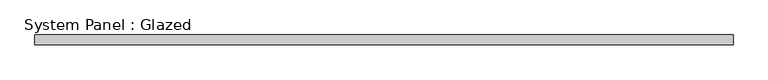
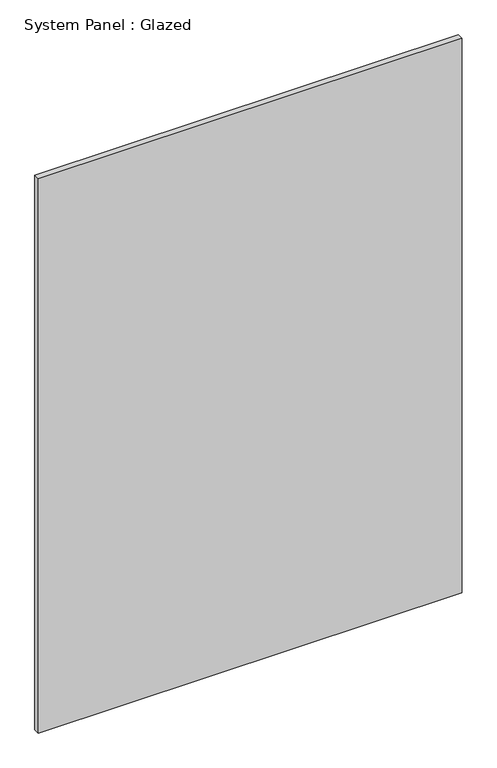
"""IFC4 building model written with IfcOpenShell, lengths in millimetres: plate geometry, System Panel : Glazed."""

from ifc_helpers import new_model, si_unit, origin, origin_with_axes, place, context, project, spatial, polyline, outline, extrude, source, transform, mapped, element, save


def system_panel_glazed_e1ffc32d(model_context):
    return source(origin(), model_context, "Body", "SweptSolid", [
        extrude(outline(polyline([(877.5, 24.5), (-877.5, 24.5), (-877.5, 49.5), (877.5, 49.5), (877.5, 24.5)])), origin_with_axes(), (0.0, 0.0, 1.0), 2425.0),
    ])


if __name__ == "__main__":
    model = new_model("IFC4")
    model_context = context("Model", 3, world=origin())
    ifc_project = project(units=[si_unit("LENGTHUNIT", "METRE", prefix="MILLI")], contexts=[model_context])
    site = spatial("IfcSite", under=ifc_project)
    building = spatial("IfcBuilding", under=site)
    placement = place(None, origin())
    system_panel_glazed_shape = system_panel_glazed_e1ffc32d(model_context)
    element("IfcPlate", 1, ObjectType="System Panel : Glazed", at=placement, inside=building, context=model_context, shape_type="MappedRepresentation", body=[
        mapped(system_panel_glazed_shape, transform((0.0, 0.0, 0.0), x_axis=(1.0, 0.0, 0.0), y_axis=(0.0, 1.0, 0.0), z_axis=(0.0, 0.0, 1.0))),
    ])
    save(model, "model.ifc")

# Revit data of these elements
# Type "System Panel : Glazed"
#   Keynote = "H11"
#   Construction Type Id = "GSP4R"
#   Analytic Construction = "1/8 in Pilkington single glazing"
#   Visual Light Transmittance = 0.9
#   Solar Heat Gain Coefficient = 0.86
#   Heat Transfer Coefficient (U) = 6.7069 W/(m²·K)
# Element 1 (IfcPlate, "System Panel : Glazed")
#   Materials on its faces: "Glass"
# Materials
#   "Glass": class "Glass", colour RGB 0 128 192, transparency 0.9, Description = "Soda Lime Glass", Cost = 0
